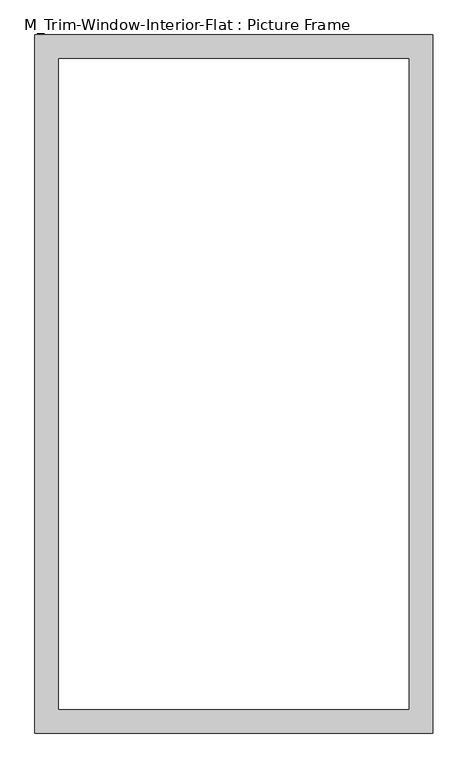
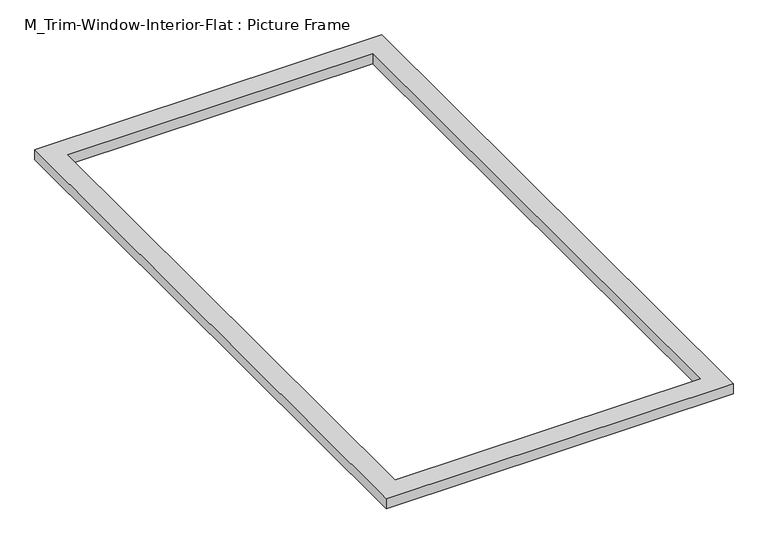
"""IFC4 building model written with IfcOpenShell, lengths in millimetres: proxy geometry, M_Trim-Window-Interior-Flat : Picture Frame."""

from ifc_helpers import new_model, si_unit, origin, origin_with_axes, place, context, project, spatial, polyline, outline, extrude, source, transform, mapped, element, save


def m_trim_window_interior_flat_picture_frame_313add5a(model_context):
    return source(origin(), model_context, "Body", "SweptSolid", [
        extrude(outline(polyline([(497.3, 47.3), (497.3, -1697.3), (-497.3, -1697.3), (-497.3, 47.3), (497.3, 47.3)]), holes=[polyline([(437.3, -12.7), (-437.3, -12.7), (-437.3, -1637.3), (437.3, -1637.3), (437.3, -12.7)])]), origin_with_axes(), (0.0, 0.0, 1.0), 30.0),
    ])


if __name__ == "__main__":
    model = new_model("IFC4")
    model_context = context("Model", 3, world=origin())
    ifc_project = project(units=[si_unit("LENGTHUNIT", "METRE", prefix="MILLI")], contexts=[model_context])
    site = spatial("IfcSite", under=ifc_project)
    building = spatial("IfcBuilding", under=site)
    placement = place(None, origin())
    m_trim_window_interior_flat_picture_frame_shape = m_trim_window_interior_flat_picture_frame_313add5a(model_context)
    element("IfcBuildingElementProxy", 1, Name="M_Trim-Window-Interior-Flat : Picture Frame", ObjectType="M_Trim-Window-Interior-Flat : Picture Frame", at=placement, inside=building, context=model_context, shape_type="MappedRepresentation", body=[
        mapped(m_trim_window_interior_flat_picture_frame_shape, transform((0.0, 0.0, 0.0), x_axis=(1.0, 0.0, 0.0), y_axis=(0.0, 1.0, 0.0), z_axis=(0.0, 0.0, 1.0))),
    ])
    save(model, "model.ifc")

# Revit data of these elements
# Type "M_Trim-Window-Interior-Flat : Picture Frame"
#   Trim Thickness_Picture Frame = 30 mm
#   Trim Width = 60 mm
#   Trim Thickness_with Sill = 20 mm
#   Sill Thickness = 30 mm
#   Opening Width [instance default] = 600 mm
#   Opening Height [instance default] = 900 mm
#   Default Elevation = 1200 mm
#   Sill = no
#   Picture Frame = yes
#   Trim Material [instance default] = none
# Element 1 (IfcBuildingElementProxy, "M_Trim-Window-Interior-Flat : Picture Frame")
#   Opening Width = 900 mm
#   Opening Height = 1650 mm
#   Trim Material = Wood - Stained
#   Materials on its faces: "Wood - Stained"
# Materials
#   "Wood - Stained": class "Wood", colour RGB 173 132 96, transparency 0, Cost = 0
